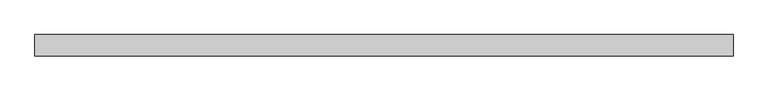
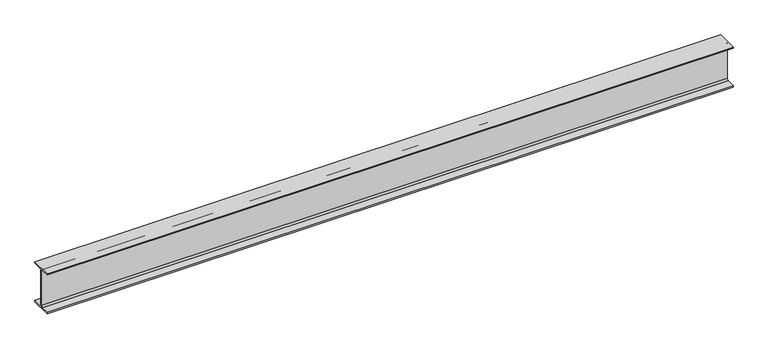
"""IFC4 building model written with IfcOpenShell, lengths in millimetres: beam geometry, 0912_Steel Framing_H-KSD3502 : H_SB_ASB_H-350x175x7x11."""

import ifcopenshell
import ifcopenshell.guid

model = None  # the IFC model being written
_history = None  # IfcOwnerHistory: only IFC2X3 demands one
_inside = {}  # id of a spatial element -> (the spatial element, [elements in it])
_under = {}  # id of a project, library or spatial element -> (it, [spatial elements below it])
_declared = {}  # id of a project -> (the project, [libraries it declares])
_typed = {}  # id of a type object -> (the type object, [elements of that type])
_made_of = {}  # id of a material, layer set ... -> (it, [elements and type objects made of it])


def new_model(schema):
    """Start an empty IFC model of exactly this schema.

    Asked for "IFC4X3", IfcOpenShell would pick the latest addendum, in which some entities
    have other attributes; the version numbers below select the first issue.
    IFC2X3 requires an IfcOwnerHistory on every rooted entity: one is made here for all.
    """
    global model, _history
    if schema == "IFC4X3":
        model = ifcopenshell.file(schema_version=(4, 3, 0, 0))
    else:
        model = ifcopenshell.file(schema=schema)
    _inside.clear()
    _under.clear()
    _declared.clear()
    _typed.clear()
    _made_of.clear()
    _history = None
    if model.schema == "IFC2X3":
        org = make("IfcOrganization", Name="unknown")
        user = make(
            "IfcPersonAndOrganization",
            ThePerson=make("IfcPerson", FamilyName="unknown"),
            TheOrganization=org,
        )
        app = make(
            "IfcApplication",
            ApplicationDeveloper=org,
            Version="unknown",
            ApplicationFullName="unknown",
            ApplicationIdentifier="unknown",
        )
        _history = make(
            "IfcOwnerHistory",
            OwningUser=user,
            OwningApplication=app,
            ChangeAction="ADDED",
            CreationDate=0,
        )
    return model


def make(cls, **values):
    """One entity of the class cls with the attributes given. An attribute that is None is left unset."""
    return model.create_entity(
        cls, **{name: value for name, value in values.items() if value is not None}
    )


def rooted(cls, **values):
    """An entity with a GlobalId (a new one), such as an element, a storey or a relation."""
    return make(cls, GlobalId=ifcopenshell.guid.new(), OwnerHistory=_history, **values)


def si_unit(unit_type, name, prefix=None):
    """IfcSIUnit, for example si_unit("LENGTHUNIT", "METRE", prefix="MILLI")."""
    return make("IfcSIUnit", UnitType=unit_type, Prefix=prefix, Name=name)


def assignment(units):
    """IfcUnitAssignment: the units of a project."""
    return None if units is None else make("IfcUnitAssignment", Units=units)


def point(xyz):
    """IfcCartesianPoint."""
    return None if xyz is None else make("IfcCartesianPoint", Coordinates=xyz)


def direction(xyz):
    """IfcDirection."""
    return None if xyz is None else make("IfcDirection", DirectionRatios=xyz)


def frame(location, z_axis=None, x_axis=None):
    """IfcAxis2Placement3D, a coordinate frame: its origin and axes. An axis left out is left unset."""
    return make(
        "IfcAxis2Placement3D",
        Location=point(location),
        Axis=direction(z_axis),
        RefDirection=direction(x_axis),
    )


def frame_2d(location, x_axis=None):
    """IfcAxis2Placement2D, a coordinate frame in the plane: its origin and x axis."""
    return make(
        "IfcAxis2Placement2D", Location=point(location), RefDirection=direction(x_axis)
    )


def origin():
    """The frame at (0, 0, 0) with its axes left unset."""
    return frame((0.0, 0.0, 0.0))


def place(relative_to, where):
    """IfcLocalPlacement: puts the frame where relative to a parent placement (None: the world)."""
    return make(
        "IfcLocalPlacement", PlacementRelTo=relative_to, RelativePlacement=where
    )


def context(
    kind, dimensions, precision=None, world=None, true_north=None, identifier=None
):
    """IfcGeometricRepresentationContext, for example the 3D "Model" context."""
    return make(
        "IfcGeometricRepresentationContext",
        ContextIdentifier=identifier,
        ContextType=kind,
        CoordinateSpaceDimension=dimensions,
        Precision=precision,
        WorldCoordinateSystem=world,
        TrueNorth=true_north,
    )


def project(units=None, contexts=None):
    """IfcProject with its units and contexts."""
    return rooted(
        "IfcProject",
        Name="project",
        RepresentationContexts=contexts,
        UnitsInContext=assignment(units),
    )


def spatial(cls, under=None, at=None, **own):
    """A site, building, storey or space (cls), placed at a placement, below another one or the project."""
    s = rooted(cls, ObjectPlacement=at, **own)
    if under is not None:
        _under.setdefault(under.id(), (under, []))[1].append(s)
    return s


def polyline(points):
    """IfcPolyline through the points."""
    return make("IfcPolyline", Points=[point(p) for p in points])


def circle_curve(where, radius):
    """IfcCircle in the frame where."""
    return make("IfcCircle", Position=where, Radius=radius)


def trimmed(basis, trim1, trim2, sense, master):
    """IfcTrimmedCurve: the piece of a basis curve between two trims."""
    return make(
        "IfcTrimmedCurve",
        BasisCurve=basis,
        Trim1=trim1,
        Trim2=trim2,
        SenseAgreement=sense,
        MasterRepresentation=master,
    )


def segment(curve, same_sense, transition):
    """IfcCompositeCurveSegment."""
    return make(
        "IfcCompositeCurveSegment",
        Transition=transition,
        SameSense=same_sense,
        ParentCurve=curve,
    )


def composite_curve(segments, self_intersect=None):
    """IfcCompositeCurve: segments joined end to end."""
    return make("IfcCompositeCurve", Segments=segments, SelfIntersect=self_intersect)


def outline(outer, holes=None, kind="AREA"):
    """IfcArbitraryClosedProfileDef: a profile drawn as a closed curve; with holes, ...WithVoids."""
    if holes is None:
        return make("IfcArbitraryClosedProfileDef", ProfileType=kind, OuterCurve=outer)
    return make(
        "IfcArbitraryProfileDefWithVoids",
        ProfileType=kind,
        OuterCurve=outer,
        InnerCurves=holes,
    )


def extrude(swept, where, along, depth):
    """IfcExtrudedAreaSolid: the profile swept, set in the frame where, extruded along a direction by depth."""
    return make(
        "IfcExtrudedAreaSolid",
        SweptArea=swept,
        Position=where,
        ExtrudedDirection=direction(along),
        Depth=depth,
    )


def shape(context_of_items, identifier, shape_type, items):
    """IfcShapeRepresentation: the items that make up one representation, for example the "Body"."""
    return make(
        "IfcShapeRepresentation",
        ContextOfItems=context_of_items,
        RepresentationIdentifier=identifier,
        RepresentationType=shape_type,
        Items=items,
    )


def source(mapping_origin, context_of_items, identifier, shape_type, items):
    """IfcRepresentationMap: a shape defined once, which mapped items show again and again."""
    return make(
        "IfcRepresentationMap",
        MappingOrigin=mapping_origin,
        MappedRepresentation=shape(context_of_items, identifier, shape_type, items),
    )


def transform(
    local_origin,
    x_axis=None,
    y_axis=None,
    z_axis=None,
    scale=None,
    scale2=None,
    scale3=None,
    uniform=True,
):
    """IfcCartesianTransformationOperator3D, or its non-uniform kind. x_axis, y_axis, z_axis: its Axis1, 2, 3."""
    if uniform:
        return make(
            "IfcCartesianTransformationOperator3D",
            Axis1=direction(x_axis),
            Axis2=direction(y_axis),
            LocalOrigin=point(local_origin),
            Scale=scale,
            Axis3=direction(z_axis),
        )
    return make(
        "IfcCartesianTransformationOperator3DnonUniform",
        Axis1=direction(x_axis),
        Axis2=direction(y_axis),
        LocalOrigin=point(local_origin),
        Scale=scale,
        Axis3=direction(z_axis),
        Scale2=scale2,
        Scale3=scale3,
    )


def mapped(mapping_source, mapping_target):
    """IfcMappedItem: shows the shape of a source again, moved by a transform."""
    return make(
        "IfcMappedItem", MappingSource=mapping_source, MappingTarget=mapping_target
    )


def made_of(thing, what):
    """Note that an element or type object is made of a material, layer set ...; save() writes the relation."""
    if what is not None:
        _made_of.setdefault(what.id(), (what, []))[1].append(thing)
    return thing


def element(
    cls,
    number,
    at=None,
    inside=None,
    cuts=None,
    type_object=None,
    material=None,
    context=None,
    identifier="Body",
    shape_type=None,
    held_by="IfcProductDefinitionShape",
    body=None,
    shapes=None,
    **own,
):
    """One element of the class cls, such as IfcWall. Its Tag is "e" and its number.

    at: its placement. inside: the storey or other place that contains it. cuts: it is an
    opening in that element (IfcRelVoidsElement). A single representation is given by context,
    identifier, shape_type and body (its items); several are given by shapes. held_by: the class
    of the entity that holds the representations. save() writes the other relations.
    """
    e = rooted(cls, Tag="e%d" % number, ObjectPlacement=at, **own)
    if body is not None:
        shapes = [shape(context, identifier, shape_type, body)]
    if shapes is not None:
        e.Representation = make(held_by, Representations=shapes)
    if inside is not None:
        _inside.setdefault(inside.id(), (inside, []))[1].append(e)
    if cuts is not None:
        rooted(
            "IfcRelVoidsElement", RelatingBuildingElement=cuts, RelatedOpeningElement=e
        )
    if type_object is not None:
        _typed.setdefault(type_object.id(), (type_object, []))[1].append(e)
    return made_of(e, material)


def aggregate(whole, parts):
    """IfcRelAggregates: a whole, such as a stair, and the parts it consists of."""
    return rooted("IfcRelAggregates", RelatingObject=whole, RelatedObjects=parts)


def save(model, path):
    """Write the relations noted so far, then the file.

    IfcRelAggregates (storeys below a building ...), IfcRelContainedInSpatialStructure (elements
    in a storey), IfcRelDefinesByType, IfcRelAssociatesMaterial and IfcRelDeclares: one each for
    every whole, place, type object, material and project.
    """
    for whole, parts in _under.values():
        aggregate(whole, parts)
    for where, things in _inside.values():
        rooted(
            "IfcRelContainedInSpatialStructure",
            RelatedElements=things,
            RelatingStructure=where,
        )
    for kind, things in _typed.values():
        rooted("IfcRelDefinesByType", RelatedObjects=things, RelatingType=kind)
    for what, things in _made_of.values():
        rooted("IfcRelAssociatesMaterial", RelatedObjects=things, RelatingMaterial=what)
    for by, libraries in _declared.values():
        rooted("IfcRelDeclares", RelatingContext=by, RelatedDefinitions=libraries)
    model.write(path)


def beam_1864dd62(model_context):
    return source(origin(), model_context, "Body", "SweptSolid", [
        extrude(outline(composite_curve([segment(polyline([(87.5, -164.0), (87.5, -175.0), (-87.5, -175.0), (-87.5, -164.0), (-17.5, -164.0)]), True, "CONTINUOUS"), segment(trimmed(circle_curve(frame_2d((-17.5, -150.0)), 14.0), [point((-17.5, -164.0))], [point((-3.5, -150.0))], True, "CARTESIAN"), True, "CONTINUOUS"), segment(polyline([(-3.5, -150.0), (-3.5, 150.0)]), True, "CONTINUOUS"), segment(trimmed(circle_curve(frame_2d((-17.5, 150.0)), 14.0), [point((-3.5, 150.0))], [point((-17.5, 164.0))], True, "CARTESIAN"), True, "CONTINUOUS"), segment(polyline([(-17.5, 164.0), (-87.5, 164.0), (-87.5, 175.0), (87.5, 175.0), (87.5, 164.0), (17.5, 164.0)]), True, "CONTINUOUS"), segment(trimmed(circle_curve(frame_2d((17.5, 150.0)), 14.0), [point((17.5, 164.0))], [point((3.5, 150.0))], True, "CARTESIAN"), True, "CONTINUOUS"), segment(polyline([(3.5, 150.0), (3.5, -150.0)]), True, "CONTINUOUS"), segment(trimmed(circle_curve(frame_2d((17.5, -150.0)), 14.0), [point((3.5, -150.0))], [point((17.5, -164.0))], True, "CARTESIAN"), True, "CONTINUOUS"), segment(polyline([(17.5, -164.0), (87.5, -164.0)]), True, "CONTINUOUS")], self_intersect=False)), frame((-2837.3, 0.0, 0.0), z_axis=(1.0, 0.0, 0.0), x_axis=(0.0, 1.0, 0.0)), (0.0, 0.0, 1.0), 5674.6),
    ])


if __name__ == "__main__":
    model = new_model("IFC4")
    model_context = context("Model", 3, world=origin())
    ifc_project = project(units=[si_unit("LENGTHUNIT", "METRE", prefix="MILLI")], contexts=[model_context])
    site = spatial("IfcSite", under=ifc_project)
    building = spatial("IfcBuilding", under=site)
    placement = place(None, origin())
    beam_shape = beam_1864dd62(model_context)
    element("IfcBeam", 1, ObjectType="0912_Steel Framing_H-KSD3502 : H_SB_ASB_H-350x175x7x11", at=placement, inside=building, context=model_context, shape_type="MappedRepresentation", body=[
        mapped(beam_shape, transform((0.0, 0.0, 0.0), x_axis=(1.0, 0.0, 0.0), y_axis=(0.0, 1.0, 0.0), z_axis=(0.0, 0.0, 1.0))),
    ])
    save(model, "model.ifc")

# Revit data of these elements
# Type "0912_Steel Framing_H-KSD3502 : H_SB_ASB_H-350x175x7x11"
#   H_WM Code_1 = "S01AA002-00001 | Main Steel Structure Fabrication Work | Shelter/Building | Medium Steel - Standard (90KG/M>Weight≥30KG/M) | Material: (   )"
#   H_WM Code_2 = "S03AA028-00001 | Main Steel Structure Erection Work | Shelter/Building | Medium Steel (90KG/M>Weight≥30KG/M) | Material: (   )"
#   H_WM Code_3 = "S01AA010-00001 | Main Steel Structure Fabrication Work | Shelter/Building | Steel Painting/Coating | for Non-Fireproofed Steel Surface, Surface Preparation, Primer, Second & Final Coat | Material: (   )"
#   H_Q'ty Cal Type Tag = "SB-Q2"
#   Width = 17.5 cm
#   Web Thickness = 0.7 cm
#   Web Fillet = 1.4 cm
#   Warping Constant = 282000.0 cm⁶
#   W = 0
#   Torsional Moment of Inertia = 19.4042 cm⁴
#   Section Area = 63.14 cm²
#   Plastic Modulus weak axis = 174.0 cm³
#   Plastic Modulus strong axis = 868.0 cm³
#   Perimeter = 1.36 m²/m
#   Nominal Weight = 49.60 kgf/m
#   Moment of Inertia weak axis = 984.00 cm⁴
#   Moment of Inertia strong axis = 13600.00 cm⁴
#   Height = 35.0 cm
#   Flange Thickness = 1.1 cm
#   Elastic Modulus weak axis = 112.0 cm³
#   Elastic Modulus strong axis = 775.0 cm³
#   Centroid Vertical = 17.5 cm
#   Centroid Horizontal = 8.75 cm
#   Ix = 136000000
#   Length [instance default] = 1.5240 m
#   Zx = 868000
#   b = 0.1750 m
#   h = 0.3500 m
#   r = 0.0140 m
#   s = 0.0070 m
#   t = 0.0110 m
#   A = 0.006314 m²
#   Structural Material [instance default] = Steel, 45-345
#   Assembly Code = ""
# Element 1 (IfcBeam, "0912_Steel Framing_H-KSD3502 : H_SB_ASB_H-350x175x7x11")
#   Structural Material = none
# Materials
#   "Steel, 45-345": class "Metal", colour RGB 189 187 185, transparency 0, Description = "Steel 345 MPa", Cost = 0
